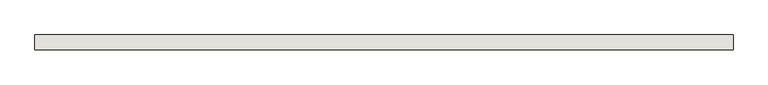
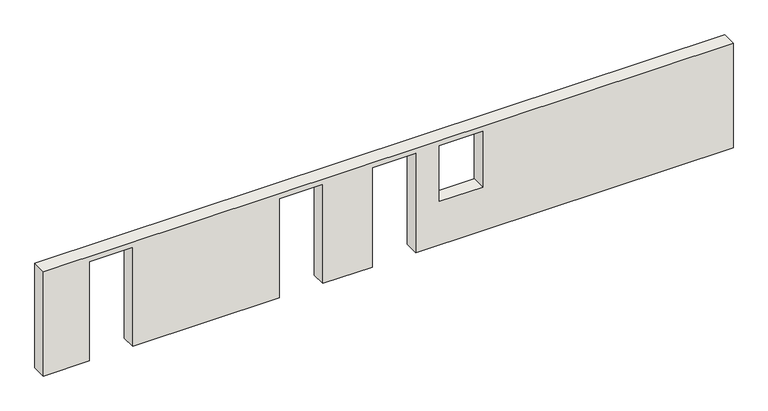
"""IFC4 building model written with IfcOpenShell, lengths in millimetres: wall geometry, 0_3d."""

import ifcopenshell
import ifcopenshell.guid

model = None  # the IFC model being written
_history = None  # IfcOwnerHistory: only IFC2X3 demands one
_inside = {}  # id of a spatial element -> (the spatial element, [elements in it])
_under = {}  # id of a project, library or spatial element -> (it, [spatial elements below it])
_declared = {}  # id of a project -> (the project, [libraries it declares])
_typed = {}  # id of a type object -> (the type object, [elements of that type])
_made_of = {}  # id of a material, layer set ... -> (it, [elements and type objects made of it])


def new_model(schema):
    """Start an empty IFC model of exactly this schema.

    Asked for "IFC4X3", IfcOpenShell would pick the latest addendum, in which some entities
    have other attributes; the version numbers below select the first issue.
    IFC2X3 requires an IfcOwnerHistory on every rooted entity: one is made here for all.
    """
    global model, _history
    if schema == "IFC4X3":
        model = ifcopenshell.file(schema_version=(4, 3, 0, 0))
    else:
        model = ifcopenshell.file(schema=schema)
    _inside.clear()
    _under.clear()
    _declared.clear()
    _typed.clear()
    _made_of.clear()
    _history = None
    if model.schema == "IFC2X3":
        org = make("IfcOrganization", Name="unknown")
        user = make(
            "IfcPersonAndOrganization",
            ThePerson=make("IfcPerson", FamilyName="unknown"),
            TheOrganization=org,
        )
        app = make(
            "IfcApplication",
            ApplicationDeveloper=org,
            Version="unknown",
            ApplicationFullName="unknown",
            ApplicationIdentifier="unknown",
        )
        _history = make(
            "IfcOwnerHistory",
            OwningUser=user,
            OwningApplication=app,
            ChangeAction="ADDED",
            CreationDate=0,
        )
    return model


def make(cls, **values):
    """One entity of the class cls with the attributes given. An attribute that is None is left unset."""
    return model.create_entity(
        cls, **{name: value for name, value in values.items() if value is not None}
    )


def rooted(cls, **values):
    """An entity with a GlobalId (a new one), such as an element, a storey or a relation."""
    return make(cls, GlobalId=ifcopenshell.guid.new(), OwnerHistory=_history, **values)


def si_unit(unit_type, name, prefix=None):
    """IfcSIUnit, for example si_unit("LENGTHUNIT", "METRE", prefix="MILLI")."""
    return make("IfcSIUnit", UnitType=unit_type, Prefix=prefix, Name=name)


def assignment(units):
    """IfcUnitAssignment: the units of a project."""
    return None if units is None else make("IfcUnitAssignment", Units=units)


def point(xyz):
    """IfcCartesianPoint."""
    return None if xyz is None else make("IfcCartesianPoint", Coordinates=xyz)


def direction(xyz):
    """IfcDirection."""
    return None if xyz is None else make("IfcDirection", DirectionRatios=xyz)


def frame(location, z_axis=None, x_axis=None):
    """IfcAxis2Placement3D, a coordinate frame: its origin and axes. An axis left out is left unset."""
    return make(
        "IfcAxis2Placement3D",
        Location=point(location),
        Axis=direction(z_axis),
        RefDirection=direction(x_axis),
    )


def origin():
    """The frame at (0, 0, 0) with its axes left unset."""
    return frame((0.0, 0.0, 0.0))


def place(relative_to, where):
    """IfcLocalPlacement: puts the frame where relative to a parent placement (None: the world)."""
    return make(
        "IfcLocalPlacement", PlacementRelTo=relative_to, RelativePlacement=where
    )


def context(
    kind, dimensions, precision=None, world=None, true_north=None, identifier=None
):
    """IfcGeometricRepresentationContext, for example the 3D "Model" context."""
    return make(
        "IfcGeometricRepresentationContext",
        ContextIdentifier=identifier,
        ContextType=kind,
        CoordinateSpaceDimension=dimensions,
        Precision=precision,
        WorldCoordinateSystem=world,
        TrueNorth=true_north,
    )


def project(units=None, contexts=None):
    """IfcProject with its units and contexts."""
    return rooted(
        "IfcProject",
        Name="project",
        RepresentationContexts=contexts,
        UnitsInContext=assignment(units),
    )


def spatial(cls, under=None, at=None, **own):
    """A site, building, storey or space (cls), placed at a placement, below another one or the project."""
    s = rooted(cls, ObjectPlacement=at, **own)
    if under is not None:
        _under.setdefault(under.id(), (under, []))[1].append(s)
    return s


def polyline(points):
    """IfcPolyline through the points."""
    return make("IfcPolyline", Points=[point(p) for p in points])


def outline(outer, holes=None, kind="AREA"):
    """IfcArbitraryClosedProfileDef: a profile drawn as a closed curve; with holes, ...WithVoids."""
    if holes is None:
        return make("IfcArbitraryClosedProfileDef", ProfileType=kind, OuterCurve=outer)
    return make(
        "IfcArbitraryProfileDefWithVoids",
        ProfileType=kind,
        OuterCurve=outer,
        InnerCurves=holes,
    )


def extrude(swept, where, along, depth):
    """IfcExtrudedAreaSolid: the profile swept, set in the frame where, extruded along a direction by depth."""
    return make(
        "IfcExtrudedAreaSolid",
        SweptArea=swept,
        Position=where,
        ExtrudedDirection=direction(along),
        Depth=depth,
    )


def shape(context_of_items, identifier, shape_type, items):
    """IfcShapeRepresentation: the items that make up one representation, for example the "Body"."""
    return make(
        "IfcShapeRepresentation",
        ContextOfItems=context_of_items,
        RepresentationIdentifier=identifier,
        RepresentationType=shape_type,
        Items=items,
    )


def source(mapping_origin, context_of_items, identifier, shape_type, items):
    """IfcRepresentationMap: a shape defined once, which mapped items show again and again."""
    return make(
        "IfcRepresentationMap",
        MappingOrigin=mapping_origin,
        MappedRepresentation=shape(context_of_items, identifier, shape_type, items),
    )


def transform(
    local_origin,
    x_axis=None,
    y_axis=None,
    z_axis=None,
    scale=None,
    scale2=None,
    scale3=None,
    uniform=True,
):
    """IfcCartesianTransformationOperator3D, or its non-uniform kind. x_axis, y_axis, z_axis: its Axis1, 2, 3."""
    if uniform:
        return make(
            "IfcCartesianTransformationOperator3D",
            Axis1=direction(x_axis),
            Axis2=direction(y_axis),
            LocalOrigin=point(local_origin),
            Scale=scale,
            Axis3=direction(z_axis),
        )
    return make(
        "IfcCartesianTransformationOperator3DnonUniform",
        Axis1=direction(x_axis),
        Axis2=direction(y_axis),
        LocalOrigin=point(local_origin),
        Scale=scale,
        Axis3=direction(z_axis),
        Scale2=scale2,
        Scale3=scale3,
    )


def mapped(mapping_source, mapping_target):
    """IfcMappedItem: shows the shape of a source again, moved by a transform."""
    return make(
        "IfcMappedItem", MappingSource=mapping_source, MappingTarget=mapping_target
    )


def made_of(thing, what):
    """Note that an element or type object is made of a material, layer set ...; save() writes the relation."""
    if what is not None:
        _made_of.setdefault(what.id(), (what, []))[1].append(thing)
    return thing


def element(
    cls,
    number,
    at=None,
    inside=None,
    cuts=None,
    type_object=None,
    material=None,
    context=None,
    identifier="Body",
    shape_type=None,
    held_by="IfcProductDefinitionShape",
    body=None,
    shapes=None,
    **own,
):
    """One element of the class cls, such as IfcWall. Its Tag is "e" and its number.

    at: its placement. inside: the storey or other place that contains it. cuts: it is an
    opening in that element (IfcRelVoidsElement). A single representation is given by context,
    identifier, shape_type and body (its items); several are given by shapes. held_by: the class
    of the entity that holds the representations. save() writes the other relations.
    """
    e = rooted(cls, Tag="e%d" % number, ObjectPlacement=at, **own)
    if body is not None:
        shapes = [shape(context, identifier, shape_type, body)]
    if shapes is not None:
        e.Representation = make(held_by, Representations=shapes)
    if inside is not None:
        _inside.setdefault(inside.id(), (inside, []))[1].append(e)
    if cuts is not None:
        rooted(
            "IfcRelVoidsElement", RelatingBuildingElement=cuts, RelatedOpeningElement=e
        )
    if type_object is not None:
        _typed.setdefault(type_object.id(), (type_object, []))[1].append(e)
    return made_of(e, material)


def aggregate(whole, parts):
    """IfcRelAggregates: a whole, such as a stair, and the parts it consists of."""
    return rooted("IfcRelAggregates", RelatingObject=whole, RelatedObjects=parts)


def save(model, path):
    """Write the relations noted so far, then the file.

    IfcRelAggregates (storeys below a building ...), IfcRelContainedInSpatialStructure (elements
    in a storey), IfcRelDefinesByType, IfcRelAssociatesMaterial and IfcRelDeclares: one each for
    every whole, place, type object, material and project.
    """
    for whole, parts in _under.values():
        aggregate(whole, parts)
    for where, things in _inside.values():
        rooted(
            "IfcRelContainedInSpatialStructure",
            RelatedElements=things,
            RelatingStructure=where,
        )
    for kind, things in _typed.values():
        rooted("IfcRelDefinesByType", RelatedObjects=things, RelatingType=kind)
    for what, things in _made_of.values():
        rooted("IfcRelAssociatesMaterial", RelatedObjects=things, RelatingMaterial=what)
    for by, libraries in _declared.values():
        rooted("IfcRelDeclares", RelatingContext=by, RelatedDefinitions=libraries)
    model.write(path)


def wall_ab64514f(model_context):
    return source(origin(), model_context, "Body", "SweptSolid", [
        extrude(outline(polyline([(0.0, 1200.0), (2740.0, 1200.0), (2740.0, 2335.0), (0.0, 2335.0), (0.0, 6160.3619019), (2740.0, 6160.3619019), (2740.0, 7295.3619019), (0.0, 7295.3619019), (0.0, 8579.9644869), (2740.0, 8579.9644869), (2740.0, 9714.9644869), (0.0, 9714.9644869), (0.0, 18002.8619019), (2880.0, 18002.8619019), (2880.0, 0.0), (0.0, 0.0), (0.0, 1200.0)]), holes=[polyline([(2740.0, 11468.674872), (1200.0, 11468.674872), (1200.0, 10333.674872), (2740.0, 10333.674872), (2740.0, 11468.674872)])]), frame((0.0, 0.0, 0.0), z_axis=(0.0, 1.0, 0.0), x_axis=(0.0, 0.0, 1.0)), (0.0, 0.0, 1.0), 380.0),
    ])


if __name__ == "__main__":
    model = new_model("IFC4")
    model_context = context("Model", 3, world=origin())
    ifc_project = project(units=[si_unit("LENGTHUNIT", "METRE", prefix="MILLI")], contexts=[model_context])
    site = spatial("IfcSite", under=ifc_project)
    building = spatial("IfcBuilding", under=site)
    placement = place(None, origin())
    wall_shape = wall_ab64514f(model_context)
    element("IfcWall", 1, ObjectType="0_3d", at=placement, inside=building, context=model_context, shape_type="MappedRepresentation", body=[
        mapped(wall_shape, transform((0.0, 0.0, 0.0), x_axis=(1.0, 0.0, 0.0), y_axis=(0.0, 1.0, 0.0), z_axis=(0.0, 0.0, 1.0))),
    ])
    save(model, "model.ifc")

# Revit data of these elements
# Element 1 (IfcWall, "0_3d")
#   Materials on its faces: "holzschalung"
# Materials
#   "holzschalung": class "Unassigned", colour RGB 128 128 128, transparency 0
